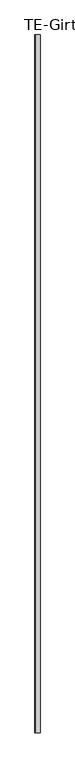
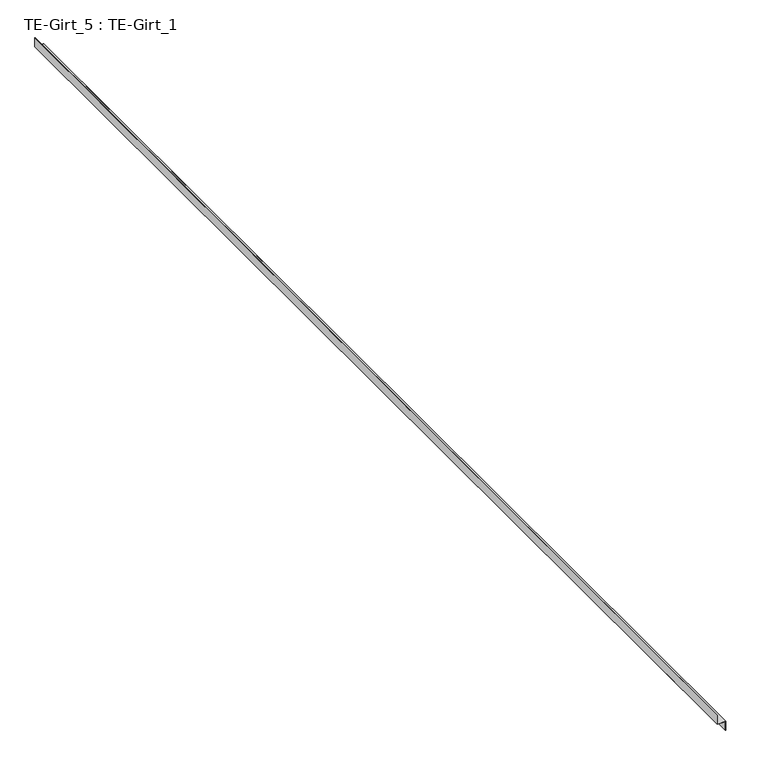
"""IFC4 building model written with IfcOpenShell, lengths in millimetres: proxy geometry, TE-Girt_5 : TE-Girt_1."""

from ifc_helpers import new_model, si_unit, frame, origin, place, context, project, spatial, polyline, outline, extrude, source, transform, mapped, element, save


def te_girt_5_te_girt_1_7c41e33f(model_context):
    return source(origin(), model_context, "Body", "SweptSolid", [
        extrude(outline(polyline([(1657.35, 590353.5520246), (1657.35, 590319.5364427), (1694.5570313, 590319.5364427), (1694.5570313, 590318.6434739), (1656.4570313, 590318.6434739), (1656.4570313, 590352.6590559), (1619.25, 590352.6590559), (1619.25, 590353.5520246), (1657.35, 590353.5520246)])), frame((0.0, -536417.5913841, 0.0), z_axis=(0.0, 1.0, 0.0), x_axis=(0.0, 0.0, 1.0)), (0.0, 0.0, 1.0), 4778.375),
    ])


if __name__ == "__main__":
    model = new_model("IFC4")
    model_context = context("Model", 3, world=origin())
    ifc_project = project(units=[si_unit("LENGTHUNIT", "METRE", prefix="MILLI")], contexts=[model_context])
    site = spatial("IfcSite", under=ifc_project)
    building = spatial("IfcBuilding", under=site)
    placement = place(None, origin())
    te_girt_5_te_girt_1_shape = te_girt_5_te_girt_1_7c41e33f(model_context)
    element("IfcBuildingElementProxy", 1, Name="TE-Girt_5 : TE-Girt_1", ObjectType="TE-Girt_5 : TE-Girt_1", at=placement, inside=building, context=model_context, shape_type="MappedRepresentation", body=[
        mapped(te_girt_5_te_girt_1_shape, transform((0.0, 0.0, 0.0), x_axis=(1.0, 0.0, 0.0), y_axis=(0.0, 1.0, 0.0), z_axis=(0.0, 0.0, 1.0))),
    ])
    save(model, "model.ifc")

# Revit data of these elements
# Element 1 (IfcBuildingElementProxy, "TE-Girt_5 : TE-Girt_1")
#   Materials on its faces: "Z-FURRING, COLD-FORMED GALV."
# Materials
#   "Z-FURRING, COLD-FORMED GALV.": class "Generic", colour RGB 143 142 141, transparency 0, Cost = 0
